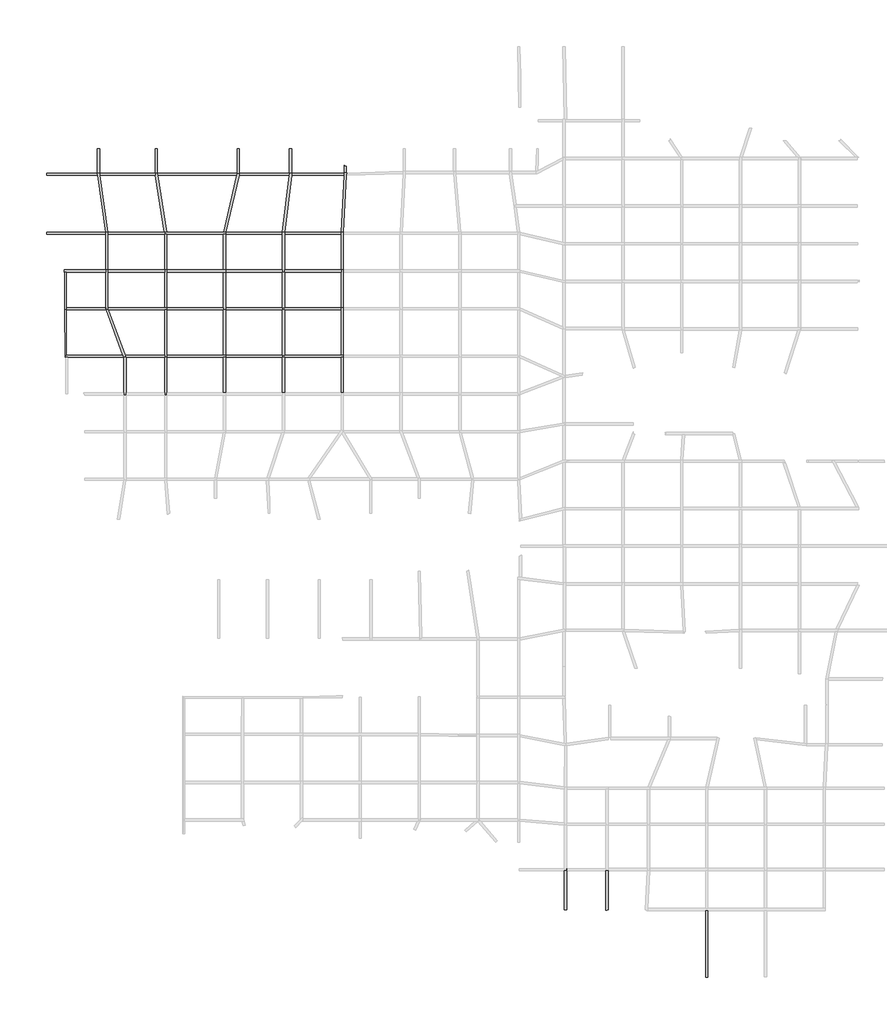
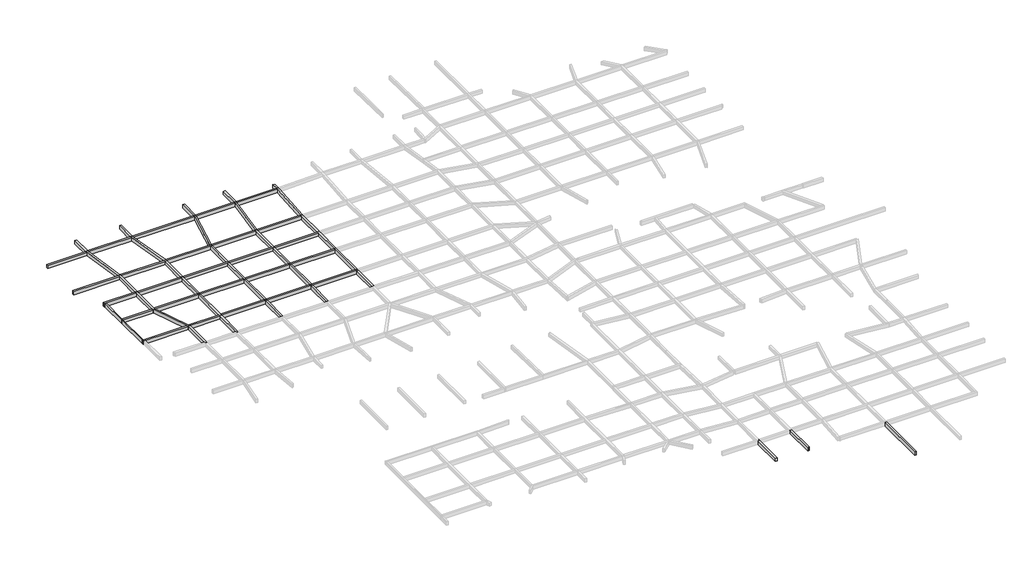
# One storey, part 2 of 15: 60 beams.
"""IFC4 building model written with IfcOpenShell, lengths in millimetres."""

from ifc_helpers import new_model, si_unit, frame, origin, place, context, project, spatial, polyline, outline, extrude, faceted_brep, element, save

model = new_model("IFC4")

# Units and contexts
model_context = context("Model", 3, world=origin())
ifc_project = project(units=[si_unit("LENGTHUNIT", "METRE", prefix="MILLI")], contexts=[model_context])

# Site, building, storey
site = spatial("IfcSite", under=ifc_project)
building = spatial("IfcBuilding", under=site)
storey = spatial("IfcBuildingStorey", under=building, Name="层高", Elevation=3300.0)

# Beams
placement = place(None, origin())
element("IfcBeam", 1, ObjectType="混凝土 - 矩形梁 : KL_beam", at=placement, inside=storey, context=model_context, shape_type="Brep", body=[
    faceted_brep([(154049.2046874, 32542.26105, 3300.0), (154049.7804968, 32392.5495084, 3300.0), (154049.7804968, 32542.26105, 3300.0), (154049.7804968, 32392.5495084, 2700.0), (154049.2046874, 32542.26105, 2700.0), (154049.7804968, 32542.26105, 2700.0)], [[[0, 1, 2]], [[3, 4, 5]], [[5, 2, 1, 3]], [[2, 5, 4, 0]], [[1, 0, 4, 3]]]),
    faceted_brep([(153749.7804968, 32242.26105, 3300.0), (153749.7804968, 32242.26105, 2700.0), (153749.7804968, 27044.9842098, 2700.0), (153749.7804968, 27044.9842098, 3300.0), (153750.3563062, 32242.26105, 3300.0), (154049.7804968, 32242.26105, 3300.0), (154049.7804968, 32242.26105, 2700.0), (153750.3563062, 32242.26105, 2700.0), (154049.7804968, 27044.9842098, 3300.0), (154049.7804968, 27044.9842098, 2700.0)], [[[0, 1, 2, 3]], [[1, 0, 4, 5, 6, 7]], [[4, 0, 3, 8, 5]], [[7, 6, 9, 2, 1]], [[6, 5, 8, 9]], [[3, 2, 9, 8]]]),
])
element("IfcBeam", 2, ObjectType="混凝土 - 矩形梁 : KL_beam", at=placement, inside=storey, context=model_context, shape_type="Brep", body=[
    faceted_brep([(159249.7804968, 32242.26105, 3300.0), (159249.7804968, 27016.5295438, 3300.0), (159372.7804968, 27016.5295438, 3300.0), (159372.7804968, 27044.9842098, 3300.0), (159492.7804968, 27044.9842098, 3300.0), (159549.7804968, 27044.9842098, 3300.0), (159549.7804968, 32242.26105, 3300.0), (159249.7804968, 27016.5295438, 2700.0), (159249.7804968, 32242.26105, 2700.0), (159549.7804968, 32242.26105, 2700.0), (159549.7804968, 27044.9842098, 2700.0), (159372.7804968, 27044.9842098, 2700.0), (159372.7804968, 27016.5295438, 2700.0)], [[[0, 1, 2, 3, 4, 5, 6]], [[7, 1, 0, 8]], [[7, 8, 9, 10, 11, 12]], [[9, 6, 5, 10]], [[0, 6, 9, 8]], [[11, 3, 2, 12]], [[3, 11, 10, 5, 4]], [[1, 7, 12, 2]]]),
])
element("IfcBeam", 3, ObjectType="混凝土 - 矩形梁 : KL_beam", at=placement, inside=storey, context=model_context, shape_type="SweptSolid", body=[
    extrude(outline(polyline([(172749.7804968, 18102.1039685), (172449.7804968, 18102.1039685), (172449.7804968, 26942.26105), (172749.7804968, 26942.26105), (172749.7804968, 18102.1039685)])), frame((0.0, 0.0, 2700.0), z_axis=(0.0, 0.0, 1.0), x_axis=(1.0, 0.0, 0.0)), (0.0, 0.0, 1.0), 600.0),
])
element("IfcBeam", 4, ObjectType="混凝土 - 矩形梁 : KL_beam", at=placement, inside=storey, context=model_context, shape_type="Brep", body=[
    faceted_brep([(92950.3009381, 106592.3894162, 3300.0), (92995.5104525, 106592.3894162, 3300.0), (93250.3009381, 106592.3894162, 3300.0), (93250.3009381, 106892.3894162, 3300.0), (93250.3009381, 111592.3894162, 3300.0), (93250.3009381, 111892.3894162, 3300.0), (92950.3009381, 111892.3894162, 3300.0), (92950.3009381, 111592.3894162, 3300.0), (92950.3009381, 106892.3894162, 3300.0), (92950.3009381, 106715.773716, 3300.0), (92950.3009381, 106592.3894162, 2700.0), (92950.3009381, 111892.3894162, 2700.0), (92950.3009381, 111592.3894162, 2700.0), (92950.3009381, 106892.3894162, 2700.0), (92950.3009381, 106715.773716, 2700.0), (93250.3009381, 106592.3894162, 2700.0), (92995.5104525, 106592.3894162, 2700.0), (93250.3009381, 111892.3894162, 2700.0), (93250.3009381, 111592.3894162, 2700.0), (93250.3009381, 106892.3894162, 2700.0)], [[[0, 1, 2, 3, 4, 5, 6, 7, 8, 9]], [[10, 0, 9, 8, 7, 6, 11, 12, 13, 14]], [[15, 16, 10, 14, 13, 12, 11, 17, 18, 19]], [[2, 15, 19, 18, 17, 5, 4, 3]], [[2, 1, 0, 10, 16, 15]], [[6, 5, 17, 11]]]),
])
element("IfcBeam", 5, ObjectType="混凝土 - 矩形梁 : KL_beam", at=placement, inside=storey, context=model_context, shape_type="Brep", body=[
    faceted_brep([(101050.3009381, 106592.3894162, 3300.0), (101050.3009381, 106892.3894162, 3300.0), (100750.3009381, 106892.3894162, 3300.0), (93250.3009381, 106892.3894162, 3300.0), (93250.3009381, 106592.3894162, 3300.0), (93315.0150877, 106592.3894162, 3300.0), (100750.3009381, 106592.3894162, 3300.0), (101050.3009381, 106592.3894162, 2700.0), (93250.3009381, 106592.3894162, 2700.0), (93315.0150877, 106592.3894162, 2700.0), (100750.3009381, 106592.3894162, 2700.0), (101050.3009381, 106892.3894162, 2700.0), (93250.3009381, 106892.3894162, 2700.0), (100750.3009381, 106892.3894162, 2700.0)], [[[0, 1, 2, 3, 4, 5, 6]], [[7, 0, 6, 5, 4, 8, 9, 10]], [[11, 7, 10, 9, 8, 12, 13]], [[1, 11, 13, 12, 3, 2]], [[4, 3, 12, 8]], [[1, 0, 7, 11]]]),
])
element("IfcBeam", 6, ObjectType="混凝土 - 矩形梁 : KL_beam", at=placement, inside=storey, context=model_context, shape_type="Brep", body=[
    faceted_brep([(101050.3009381, 111892.3894162, 3300.0), (100750.3009381, 111892.3894162, 3300.0), (100750.3009381, 111592.3894162, 3300.0), (100750.3009381, 106892.3894162, 3300.0), (101050.3009381, 106892.3894162, 3300.0), (101050.3009381, 111592.3894162, 3300.0), (101050.3009381, 111892.3894162, 2700.0), (101050.3009381, 106892.3894162, 2700.0), (101050.3009381, 111592.3894162, 2700.0), (100750.3009381, 111892.3894162, 2700.0), (100750.3009381, 106892.3894162, 2700.0), (100750.3009381, 111592.3894162, 2700.0)], [[[0, 1, 2, 3, 4, 5]], [[6, 0, 5, 4, 7, 8]], [[9, 6, 8, 7, 10, 11]], [[1, 9, 11, 10, 3, 2]], [[4, 3, 10, 7]], [[1, 0, 6, 9]]]),
])
element("IfcBeam", 7, ObjectType="混凝土 - 矩形梁 : KL_beam", at=placement, inside=storey, context=model_context, shape_type="SweptSolid", body=[
    extrude(outline(polyline([(93250.3009381, 111592.3894162), (93250.3009381, 111892.3894162), (100750.3009381, 111892.3894162), (100750.3009381, 111592.3894162), (93250.3009381, 111592.3894162)])), frame((0.0, 0.0, 2700.0), z_axis=(0.0, 0.0, 1.0), x_axis=(1.0, 0.0, 0.0)), (0.0, 0.0, 1.0), 600.0),
])
element("IfcBeam", 8, ObjectType="混凝土 - 矩形梁 : KL_beam", at=placement, inside=storey, context=model_context, shape_type="Brep", body=[
    faceted_brep([(108850.3009381, 111592.3894162, 3300.0), (108850.3009381, 111892.3894162, 3300.0), (108550.3009381, 111892.3894162, 3300.0), (101050.3009381, 111892.3894162, 3300.0), (101050.3009381, 111592.3894162, 3300.0), (108550.3009381, 111592.3894162, 3300.0), (108850.3009381, 111592.3894162, 2700.0), (101050.3009381, 111592.3894162, 2700.0), (108550.3009381, 111592.3894162, 2700.0), (108850.3009381, 111892.3894162, 2700.0), (101050.3009381, 111892.3894162, 2700.0), (108550.3009381, 111892.3894162, 2700.0)], [[[0, 1, 2, 3, 4, 5]], [[6, 0, 5, 4, 7, 8]], [[9, 6, 8, 7, 10, 11]], [[1, 9, 11, 10, 3, 2]], [[4, 3, 10, 7]], [[1, 0, 6, 9]]]),
])
element("IfcBeam", 9, ObjectType="混凝土 - 矩形梁 : KL_beam", at=placement, inside=storey, context=model_context, shape_type="Brep", body=[
    faceted_brep([(108550.3009381, 106592.3894162, 3300.0), (108850.3009381, 106592.3894162, 3300.0), (108850.3009381, 106892.3894162, 3300.0), (108850.3009381, 111592.3894162, 3300.0), (108550.3009381, 111592.3894162, 3300.0), (108550.3009381, 106892.3894162, 3300.0), (108550.3009381, 106592.3894162, 2700.0), (108550.3009381, 111592.3894162, 2700.0), (108550.3009381, 106892.3894162, 2700.0), (108850.3009381, 106592.3894162, 2700.0), (108850.3009381, 111592.3894162, 2700.0), (108850.3009381, 106892.3894162, 2700.0)], [[[0, 1, 2, 3, 4, 5]], [[6, 0, 5, 4, 7, 8]], [[9, 6, 8, 7, 10, 11]], [[1, 9, 11, 10, 3, 2]], [[4, 3, 10, 7]], [[1, 0, 6, 9]]]),
])
element("IfcBeam", 10, ObjectType="混凝土 - 矩形梁 : KL_beam", at=placement, inside=storey, context=model_context, shape_type="SweptSolid", body=[
    extrude(outline(polyline([(101050.3009381, 106592.3894162), (101050.3009381, 106892.3894162), (108550.3009381, 106892.3894162), (108550.3009381, 106592.3894162), (101050.3009381, 106592.3894162)])), frame((0.0, 0.0, 2700.0), z_axis=(0.0, 0.0, 1.0), x_axis=(1.0, 0.0, 0.0)), (0.0, 0.0, 1.0), 600.0),
])
element("IfcBeam", 11, ObjectType="混凝土 - 矩形梁 : KL_beam", at=placement, inside=storey, context=model_context, shape_type="Brep", body=[
    faceted_brep([(100750.3009381, 100292.3894162, 3300.0), (101050.3009381, 100292.3894162, 3300.0), (101050.3009381, 100592.3894162, 3300.0), (101050.3009381, 106592.3894162, 3300.0), (100750.3009381, 106592.3894162, 3300.0), (100750.3009381, 100592.3894162, 3300.0), (101050.3009381, 100292.3894162, 2700.0), (101050.3009381, 100592.3894162, 2700.0), (101050.3009381, 106592.3894162, 2700.0), (100750.3009381, 100292.3894162, 2700.0), (100750.3009381, 100592.3894162, 2700.0), (100750.3009381, 106592.3894162, 2700.0)], [[[0, 1, 2, 3, 4, 5]], [[1, 6, 7, 8, 3, 2]], [[6, 9, 10, 11, 8, 7]], [[9, 0, 5, 4, 11, 10]], [[4, 3, 8, 11]], [[1, 0, 9, 6]]]),
])
element("IfcBeam", 12, ObjectType="混凝土 - 矩形梁 : KL_beam", at=placement, inside=storey, context=model_context, shape_type="Brep", body=[
    faceted_brep([(92950.3009381, 106715.773716, 3300.0), (92950.3009381, 106892.3894162, 3300.0), (92885.5867885, 106892.3894162, 3300.0), (92950.3009381, 106892.3894162, 2700.0), (92950.3009381, 106715.773716, 2700.0), (92885.5867885, 106892.3894162, 2700.0)], [[[0, 1, 2]], [[3, 4, 5]], [[2, 5, 4, 0]], [[5, 2, 1, 3]], [[1, 0, 4, 3]]]),
    faceted_brep([(95623.4120324, 100292.3894162, 3300.0), (95623.4120324, 100292.3894162, 2700.0), (95513.4883684, 100592.3894162, 2700.0), (93315.0150877, 106592.3894162, 2700.0), (93315.0150877, 106592.3894162, 3300.0), (95513.4883684, 100592.3894162, 3300.0), (93250.3009381, 106592.3894162, 2700.0), (92995.5104525, 106592.3894162, 2700.0), (92995.5104525, 106592.3894162, 3300.0), (93250.3009381, 106592.3894162, 3300.0), (95350.3009362, 100292.3894162, 3300.0), (95303.9073972, 100292.3894162, 3300.0), (95303.9073972, 100292.3894162, 2700.0), (95350.3009362, 100292.3894162, 2700.0), (95193.9837332, 100592.3894162, 3300.0), (95193.9837332, 100592.3894162, 2700.0)], [[[0, 1, 2, 3, 4, 5]], [[4, 3, 6, 7, 8, 9]], [[0, 10, 11, 12, 13, 1]], [[4, 9, 8, 14, 11, 10, 0, 5]], [[7, 6, 3, 2, 1, 13, 12, 15]], [[8, 7, 15, 12, 11, 14]]]),
])
element("IfcBeam", 13, ObjectType="混凝土 - 矩形梁 : KL_beam", at=placement, inside=storey, context=model_context, shape_type="Brep", body=[
    faceted_brep([(100750.3009381, 100292.3894162, 3300.0), (100750.3009381, 100592.3894162, 3300.0), (95513.4883684, 100592.3894162, 3300.0), (95623.4120324, 100292.3894162, 3300.0), (95650.3009362, 100292.3894162, 3300.0), (100750.3009381, 100292.3894162, 2700.0), (95623.4120324, 100292.3894162, 2700.0), (95650.3009362, 100292.3894162, 2700.0), (100750.3009381, 100592.3894162, 2700.0), (95513.4883684, 100592.3894162, 2700.0)], [[[0, 1, 2, 3, 4]], [[5, 0, 4, 3, 6, 7]], [[8, 5, 7, 6, 9]], [[1, 8, 9, 2]], [[1, 0, 5, 8]], [[3, 2, 9, 6]]]),
])
element("IfcBeam", 14, ObjectType="混凝土 - 矩形梁 : KL_beam", at=placement, inside=storey, context=model_context, shape_type="Brep", body=[
    faceted_brep([(108850.3009381, 100292.3894162, 3300.0), (108850.3009381, 100592.3894162, 3300.0), (108550.3009381, 100592.3894162, 3300.0), (101050.3009381, 100592.3894162, 3300.0), (101050.3009381, 100292.3894162, 3300.0), (108550.3009381, 100292.3894162, 3300.0), (108850.3009381, 100592.3894162, 2700.0), (108550.3009381, 100592.3894162, 2700.0), (101050.3009381, 100592.3894162, 2700.0), (108850.3009381, 100292.3894162, 2700.0), (108550.3009381, 100292.3894162, 2700.0), (101050.3009381, 100292.3894162, 2700.0)], [[[0, 1, 2, 3, 4, 5]], [[1, 6, 7, 8, 3, 2]], [[6, 9, 10, 11, 8, 7]], [[9, 0, 5, 4, 11, 10]], [[4, 3, 8, 11]], [[1, 0, 9, 6]]]),
])
element("IfcBeam", 15, ObjectType="混凝土 - 矩形梁 : KL_beam", at=placement, inside=storey, context=model_context, shape_type="SweptSolid", body=[
    extrude(outline(polyline([(108550.3009381, 106592.3894162), (108850.3009381, 106592.3894162), (108850.3009381, 100592.3894162), (108550.3009381, 100592.3894162), (108550.3009381, 106592.3894162)])), frame((0.0, 0.0, 2700.0), z_axis=(0.0, 0.0, 1.0), x_axis=(1.0, 0.0, 0.0)), (0.0, 0.0, 1.0), 600.0),
])
element("IfcBeam", 16, ObjectType="混凝土 - 矩形梁 : KL_beam", at=placement, inside=storey, context=model_context, shape_type="Brep", body=[
    faceted_brep([(100750.3009381, 95292.1233035, 3300.0), (101050.3009381, 95292.1233035, 3300.0), (101050.3009381, 95592.1233035, 3300.0), (101050.3009381, 100292.3894162, 3300.0), (100750.3009381, 100292.3894162, 3300.0), (100750.3009381, 95592.1233035, 3300.0), (101050.3009381, 95292.1233035, 2700.0), (101050.3009381, 95592.1233035, 2700.0), (101050.3009381, 100292.3894162, 2700.0), (100750.3009381, 95292.1233035, 2700.0), (100750.3009381, 95592.1233035, 2700.0), (100750.3009381, 100292.3894162, 2700.0)], [[[0, 1, 2, 3, 4, 5]], [[1, 6, 7, 8, 3, 2]], [[6, 9, 10, 11, 8, 7]], [[9, 0, 5, 4, 11, 10]], [[4, 3, 8, 11]], [[1, 0, 9, 6]]]),
])
element("IfcBeam", 17, ObjectType="混凝土 - 矩形梁 : KL_beam", at=placement, inside=storey, context=model_context, shape_type="Brep", body=[
    faceted_brep([(95350.3009362, 95292.1233035, 3300.0), (95650.3009362, 95292.1233035, 3300.0), (95650.3009362, 95592.1233035, 3300.0), (95650.3009362, 100292.3894162, 3300.0), (95623.4120324, 100292.3894162, 3300.0), (95350.3009362, 100292.3894162, 3300.0), (95350.3009362, 95567.3846604, 3300.0), (95650.3009362, 95292.1233035, 2700.0), (95650.3009362, 95592.1233035, 2700.0), (95650.3009362, 100292.3894162, 2700.0), (95350.3009362, 95292.1233035, 2700.0), (95350.3009362, 95567.3846604, 2700.0), (95350.3009362, 100292.3894162, 2700.0), (95623.4120324, 100292.3894162, 2700.0)], [[[0, 1, 2, 3, 4, 5, 6]], [[1, 7, 8, 9, 3, 2]], [[7, 10, 11, 12, 13, 9, 8]], [[10, 0, 6, 5, 12, 11]], [[5, 4, 3, 9, 13, 12]], [[1, 0, 10, 7]]]),
])
element("IfcBeam", 18, ObjectType="混凝土 - 矩形梁 : KL_beam", at=placement, inside=storey, context=model_context, shape_type="SweptSolid", body=[
    extrude(outline(polyline([(108550.3009381, 100292.3894162), (108850.3009381, 100292.3894162), (108850.3009381, 95592.1233035), (108550.3009381, 95592.1233035), (108550.3009381, 100292.3894162)])), frame((0.0, 0.0, 2700.0), z_axis=(0.0, 0.0, 1.0), x_axis=(1.0, 0.0, 0.0)), (0.0, 0.0, 1.0), 600.0),
])
element("IfcBeam", 19, ObjectType="混凝土 - 矩形梁 : KL_beam", at=placement, inside=storey, context=model_context, shape_type="Brep", body=[
    faceted_brep([(87611.9695307, 100592.3894162, 3300.0), (87614.7715216, 100292.3894162, 3300.0), (87650.3009381, 100292.3894162, 3300.0), (87950.3009381, 100292.3894162, 3300.0), (95303.9073972, 100292.3894162, 3300.0), (95193.9837332, 100592.3894162, 3300.0), (87750.3009381, 100592.3894162, 3300.0), (87611.9695307, 100592.3894162, 2700.0), (95193.9837332, 100592.3894162, 2700.0), (87750.3009381, 100592.3894162, 2700.0), (87614.7715216, 100292.3894162, 2700.0), (95303.9073972, 100292.3894162, 2700.0), (87950.3009381, 100292.3894162, 2700.0), (87650.3009381, 100292.3894162, 2700.0)], [[[0, 1, 2, 3, 4, 5, 6]], [[7, 0, 6, 5, 8, 9]], [[10, 7, 9, 8, 11, 12, 13]], [[1, 10, 13, 12, 11, 4, 3, 2]], [[1, 0, 7, 10]], [[5, 4, 11, 8]]]),
])
element("IfcBeam", 20, ObjectType="混凝土 - 矩形梁 : KL_beam", at=placement, inside=storey, context=model_context, shape_type="Brep", body=[
    faceted_brep([(124450.3009381, 100292.3894162, 3300.0), (124450.3009381, 100592.3894162, 3300.0), (124150.3009381, 100592.3894162, 3300.0), (116650.3009381, 100592.3894162, 3300.0), (116350.3009381, 100592.3894162, 3300.0), (116350.3009381, 100292.3894162, 3300.0), (116650.3009381, 100292.3894162, 3300.0), (124150.3009381, 100292.3894162, 3300.0), (124450.3009381, 100292.3894162, 2700.0), (116350.3009381, 100292.3894162, 2700.0), (116650.3009381, 100292.3894162, 2700.0), (124150.3009381, 100292.3894162, 2700.0), (124450.3009381, 100592.3894162, 2700.0), (116350.3009381, 100592.3894162, 2700.0), (116650.3009381, 100592.3894162, 2700.0), (124150.3009381, 100592.3894162, 2700.0)], [[[0, 1, 2, 3, 4, 5, 6, 7]], [[8, 0, 7, 6, 5, 9, 10, 11]], [[12, 8, 11, 10, 9, 13, 14, 15]], [[1, 12, 15, 14, 13, 4, 3, 2]], [[1, 0, 8, 12]], [[5, 4, 13, 9]]]),
])
element("IfcBeam", 21, ObjectType="混凝土 - 矩形梁 : KL_beam", at=placement, inside=storey, context=model_context, shape_type="Brep", body=[
    faceted_brep([(124450.3009381, 106892.3894162, 3300.0), (124150.3009381, 106892.3894162, 3300.0), (124150.3009381, 106592.3894162, 3300.0), (124150.3009381, 100592.3894162, 3300.0), (124450.3009381, 100592.3894162, 3300.0), (124450.3009381, 106592.3894162, 3300.0), (124450.3009381, 106892.3894162, 2700.0), (124450.3009381, 100592.3894162, 2700.0), (124450.3009381, 106592.3894162, 2700.0), (124150.3009381, 106892.3894162, 2700.0), (124150.3009381, 100592.3894162, 2700.0), (124150.3009381, 106592.3894162, 2700.0)], [[[0, 1, 2, 3, 4, 5]], [[6, 0, 5, 4, 7, 8]], [[9, 6, 8, 7, 10, 11]], [[1, 9, 11, 10, 3, 2]], [[4, 3, 10, 7]], [[1, 0, 6, 9]]]),
])
element("IfcBeam", 22, ObjectType="混凝土 - 矩形梁 : KL_beam", at=placement, inside=storey, context=model_context, shape_type="Brep", body=[
    faceted_brep([(116350.3009381, 106892.3894162, 3300.0), (116350.3009381, 106592.3894162, 3300.0), (116650.3009381, 106592.3894162, 3300.0), (124150.3009381, 106592.3894162, 3300.0), (124150.3009381, 106892.3894162, 3300.0), (116650.3009381, 106892.3894162, 3300.0), (116350.3009381, 106892.3894162, 2700.0), (124150.3009381, 106892.3894162, 2700.0), (116650.3009381, 106892.3894162, 2700.0), (116350.3009381, 106592.3894162, 2700.0), (124150.3009381, 106592.3894162, 2700.0), (116650.3009381, 106592.3894162, 2700.0)], [[[0, 1, 2, 3, 4, 5]], [[6, 0, 5, 4, 7, 8]], [[9, 6, 8, 7, 10, 11]], [[1, 9, 11, 10, 3, 2]], [[4, 3, 10, 7]], [[1, 0, 6, 9]]]),
])
element("IfcBeam", 23, ObjectType="混凝土 - 矩形梁 : KL_beam", at=placement, inside=storey, context=model_context, shape_type="SweptSolid", body=[
    extrude(outline(polyline([(116650.3009381, 100592.3894162), (116350.3009381, 100592.3894162), (116350.3009381, 106592.3894162), (116650.3009381, 106592.3894162), (116650.3009381, 100592.3894162)])), frame((0.0, 0.0, 2700.0), z_axis=(0.0, 0.0, 1.0), x_axis=(1.0, 0.0, 0.0)), (0.0, 0.0, 1.0), 600.0),
])
element("IfcBeam", 24, ObjectType="混凝土 - 矩形梁 : KL_beam", at=placement, inside=storey, context=model_context, shape_type="SweptSolid", body=[
    extrude(outline(polyline([(116350.3009381, 100292.3894162), (116650.3009381, 100292.3894162), (116650.3009381, 95592.1233035), (116350.3009381, 95592.1233035), (116350.3009381, 100292.3894162)])), frame((0.0, 0.0, 2700.0), z_axis=(0.0, 0.0, 1.0), x_axis=(1.0, 0.0, 0.0)), (0.0, 0.0, 1.0), 600.0),
])
element("IfcBeam", 25, ObjectType="混凝土 - 矩形梁 : KL_beam", at=placement, inside=storey, context=model_context, shape_type="SweptSolid", body=[
    extrude(outline(polyline([(124150.3009381, 100292.3894162), (124450.3009381, 100292.3894162), (124450.3009381, 95592.1233035), (124150.3009381, 95592.1233035), (124150.3009381, 100292.3894162)])), frame((0.0, 0.0, 2700.0), z_axis=(0.0, 0.0, 1.0), x_axis=(1.0, 0.0, 0.0)), (0.0, 0.0, 1.0), 600.0),
])
element("IfcBeam", 26, ObjectType="混凝土 - 矩形梁 : KL_beam", at=placement, inside=storey, context=model_context, shape_type="Brep", body=[
    faceted_brep([(116350.3009381, 111592.3894162, 3300.0), (116650.3009381, 111592.3894162, 3300.0), (116650.3009381, 111892.3894162, 3300.0), (116650.3009381, 116592.3894162, 3300.0), (116650.3009381, 116892.3894162, 3300.0), (116367.5921484, 116892.3894162, 3300.0), (116350.3009381, 116892.3894162, 3300.0), (116350.3009381, 116592.3894162, 3300.0), (116350.3009381, 111892.3894162, 3300.0), (116350.3009381, 111592.3894162, 2700.0), (116350.3009381, 116892.3894162, 2700.0), (116350.3009381, 116592.3894162, 2700.0), (116350.3009381, 111892.3894162, 2700.0), (116650.3009381, 111592.3894162, 2700.0), (116367.5921484, 116892.3894162, 2700.0), (116650.3009381, 116892.3894162, 2700.0), (116650.3009381, 116592.3894162, 2700.0), (116650.3009381, 111892.3894162, 2700.0)], [[[0, 1, 2, 3, 4, 5, 6, 7, 8]], [[9, 0, 8, 7, 6, 10, 11, 12]], [[13, 9, 12, 11, 10, 14, 15, 16, 17]], [[1, 13, 17, 16, 15, 4, 3, 2]], [[1, 0, 9, 13]], [[6, 5, 4, 15, 14, 10]]]),
])
element("IfcBeam", 27, ObjectType="混凝土 - 矩形梁 : KL_beam", at=placement, inside=storey, context=model_context, shape_type="SweptSolid", body=[
    extrude(outline(polyline([(116650.3009381, 106892.3894162), (116350.3009381, 106892.3894162), (116350.3009381, 111592.3894162), (116650.3009381, 111592.3894162), (116650.3009381, 106892.3894162)])), frame((0.0, 0.0, 2700.0), z_axis=(0.0, 0.0, 1.0), x_axis=(1.0, 0.0, 0.0)), (0.0, 0.0, 1.0), 600.0),
])
element("IfcBeam", 28, ObjectType="混凝土 - 矩形梁 : KL_beam", at=placement, inside=storey, context=model_context, shape_type="Brep", body=[
    faceted_brep([(124450.3009381, 111892.3894162, 3300.0), (124150.3009381, 111892.3894162, 3300.0), (124150.3009381, 111592.3894162, 3300.0), (124150.3009381, 106892.3894162, 3300.0), (124450.3009381, 106892.3894162, 3300.0), (124450.3009381, 111592.3894162, 3300.0), (124150.3009381, 111892.3894162, 2700.0), (124150.3009381, 111592.3894162, 2700.0), (124150.3009381, 106892.3894162, 2700.0), (124450.3009381, 111892.3894162, 2700.0), (124450.3009381, 111592.3894162, 2700.0), (124450.3009381, 106892.3894162, 2700.0)], [[[0, 1, 2, 3, 4, 5]], [[1, 6, 7, 8, 3, 2]], [[6, 9, 10, 11, 8, 7]], [[9, 0, 5, 4, 11, 10]], [[4, 3, 8, 11]], [[1, 0, 9, 6]]]),
])
element("IfcBeam", 29, ObjectType="混凝土 - 矩形梁 : KL_beam", at=placement, inside=storey, context=model_context, shape_type="SweptSolid", body=[
    extrude(outline(polyline([(116650.3009381, 111592.3894162), (116650.3009381, 111892.3894162), (124150.3009381, 111892.3894162), (124150.3009381, 111592.3894162), (116650.3009381, 111592.3894162)])), frame((0.0, 0.0, 2700.0), z_axis=(0.0, 0.0, 1.0), x_axis=(1.0, 0.0, 0.0)), (0.0, 0.0, 1.0), 600.0),
])
element("IfcBeam", 30, ObjectType="混凝土 - 矩形梁 : KL_beam", at=placement, inside=storey, context=model_context, shape_type="Brep", body=[
    faceted_brep([(124450.3009381, 116892.3894162, 3300.0), (124157.9562531, 116892.3894162, 3300.0), (124150.3009381, 116892.3894162, 3300.0), (124150.3009381, 116592.3894162, 3300.0), (124150.3009381, 111892.3894162, 3300.0), (124450.3009381, 111892.3894162, 3300.0), (124450.3009381, 116592.3894162, 3300.0), (124450.3009381, 116738.461528, 3300.0), (124450.3009381, 116892.3894162, 2700.0), (124450.3009381, 111892.3894162, 2700.0), (124450.3009381, 116592.3894162, 2700.0), (124450.3009381, 116738.461528, 2700.0), (124150.3009381, 116892.3894162, 2700.0), (124157.9562531, 116892.3894162, 2700.0), (124150.3009381, 111892.3894162, 2700.0), (124150.3009381, 116592.3894162, 2700.0)], [[[0, 1, 2, 3, 4, 5, 6, 7]], [[8, 0, 7, 6, 5, 9, 10, 11]], [[12, 13, 8, 11, 10, 9, 14, 15]], [[2, 12, 15, 14, 4, 3]], [[5, 4, 14, 9]], [[2, 1, 0, 8, 13, 12]]]),
])
element("IfcBeam", 31, ObjectType="混凝土 - 矩形梁 : KL_beam", at=placement, inside=storey, context=model_context, shape_type="Brep", body=[
    faceted_brep([(116650.3009381, 116892.3894162, 3300.0), (116650.3009381, 116592.3894162, 3300.0), (124150.3009381, 116592.3894162, 3300.0), (124150.3009381, 116892.3894162, 3300.0), (116669.8450961, 116892.3894162, 3300.0), (116650.3009381, 116892.3894162, 2700.0), (124150.3009381, 116892.3894162, 2700.0), (116669.8450961, 116892.3894162, 2700.0), (116650.3009381, 116592.3894162, 2700.0), (124150.3009381, 116592.3894162, 2700.0)], [[[0, 1, 2, 3, 4]], [[5, 0, 4, 3, 6, 7]], [[8, 5, 7, 6, 9]], [[1, 8, 9, 2]], [[1, 0, 5, 8]], [[3, 2, 9, 6]]]),
])
element("IfcBeam", 32, ObjectType="混凝土 - 矩形梁 : KL_beam", at=placement, inside=storey, context=model_context, shape_type="Brep", body=[
    faceted_brep([(100750.3009381, 116892.3894162, 3300.0), (100750.3009381, 116592.3894162, 3300.0), (101050.3009381, 116592.3894162, 3300.0), (108550.3009381, 116592.3894162, 3300.0), (108850.3009381, 116592.3894162, 3300.0), (108850.3009381, 116892.3894162, 3300.0), (108580.9855506, 116892.3894162, 3300.0), (101028.4130409, 116892.3894162, 3300.0), (100750.3009381, 116592.3894162, 2700.0), (101050.3009381, 116592.3894162, 2700.0), (108550.3009381, 116592.3894162, 2700.0), (108850.3009381, 116592.3894162, 2700.0), (100750.3009381, 116892.3894162, 2700.0), (101028.4130409, 116892.3894162, 2700.0), (108580.9855506, 116892.3894162, 2700.0), (108850.3009381, 116892.3894162, 2700.0)], [[[0, 1, 2, 3, 4, 5, 6, 7]], [[1, 8, 9, 10, 11, 4, 3, 2]], [[8, 12, 13, 14, 15, 11, 10, 9]], [[12, 0, 7, 6, 5, 15, 14, 13]], [[1, 0, 12, 8]], [[5, 4, 11, 15]]]),
])
element("IfcBeam", 33, ObjectType="混凝土 - 矩形梁 : KL_beam", at=placement, inside=storey, context=model_context, shape_type="SweptSolid", body=[
    extrude(outline(polyline([(101050.3009381, 111892.3894162), (100750.3009381, 111892.3894162), (100750.3009381, 116592.3894162), (101050.3009381, 116592.3894162), (101050.3009381, 111892.3894162)])), frame((0.0, 0.0, 2700.0), z_axis=(0.0, 0.0, 1.0), x_axis=(1.0, 0.0, 0.0)), (0.0, 0.0, 1.0), 600.0),
])
element("IfcBeam", 34, ObjectType="混凝土 - 矩形梁 : KL_beam", at=placement, inside=storey, context=model_context, shape_type="SweptSolid", body=[
    extrude(outline(polyline([(108850.3009381, 111892.3894162), (108550.3009381, 111892.3894162), (108550.3009381, 116592.3894162), (108850.3009381, 116592.3894162), (108850.3009381, 111892.3894162)])), frame((0.0, 0.0, 2700.0), z_axis=(0.0, 0.0, 1.0), x_axis=(1.0, 0.0, 0.0)), (0.0, 0.0, 1.0), 600.0),
])
element("IfcBeam", 35, ObjectType="混凝土 - 矩形梁 : KL_beam", at=placement, inside=storey, context=model_context, shape_type="Brep", body=[
    faceted_brep([(93250.3009381, 116892.3894162, 3300.0), (93230.6939488, 116892.3894162, 3300.0), (92950.3009381, 116892.3894162, 3300.0), (92950.3009381, 116592.3894162, 3300.0), (92950.3009381, 111892.3894162, 3300.0), (93250.3009381, 111892.3894162, 3300.0), (93250.3009381, 116592.3894162, 3300.0), (92950.3009381, 116892.3894162, 2700.0), (92950.3009381, 116592.3894162, 2700.0), (92950.3009381, 111892.3894162, 2700.0), (93230.6939488, 116892.3894162, 2700.0), (93250.3009381, 116892.3894162, 2700.0), (93250.3009381, 116592.3894162, 2700.0), (93250.3009381, 111892.3894162, 2700.0)], [[[0, 1, 2, 3, 4, 5, 6]], [[2, 7, 8, 9, 4, 3]], [[7, 10, 11, 12, 13, 9, 8]], [[11, 0, 6, 5, 13, 12]], [[5, 4, 9, 13]], [[2, 1, 0, 11, 10, 7]]]),
])
element("IfcBeam", 36, ObjectType="混凝土 - 矩形梁 : KL_beam", at=placement, inside=storey, context=model_context, shape_type="Brep", body=[
    faceted_brep([(100750.3009381, 116592.3894162, 3300.0), (100750.3009381, 116892.3894162, 3300.0), (100724.6735032, 116892.3894162, 3300.0), (93250.3009381, 116892.3894162, 3300.0), (93250.3009381, 116592.3894162, 3300.0), (100750.3009381, 116592.3894162, 2700.0), (93250.3009381, 116592.3894162, 2700.0), (100750.3009381, 116892.3894162, 2700.0), (93250.3009381, 116892.3894162, 2700.0), (100724.6735032, 116892.3894162, 2700.0)], [[[0, 1, 2, 3, 4]], [[5, 0, 4, 6]], [[7, 5, 6, 8, 9]], [[1, 7, 9, 8, 3, 2]], [[1, 0, 5, 7]], [[4, 3, 8, 6]]]),
])
element("IfcBeam", 37, ObjectType="混凝土 - 矩形梁 : KL_beam", at=placement, inside=storey, context=model_context, shape_type="Brep", body=[
    faceted_brep([(87450.3009381, 111892.3894162, 3300.0), (87450.3009381, 111592.3894162, 3300.0), (87750.3009381, 111592.3894162, 3300.0), (92950.3009381, 111592.3894162, 3300.0), (92950.3009381, 111892.3894162, 3300.0), (87450.3009381, 111892.3894162, 2700.0), (92950.3009381, 111892.3894162, 2700.0), (87450.3009381, 111592.3894162, 2700.0), (92950.3009381, 111592.3894162, 2700.0), (87750.3009381, 111592.3894162, 2700.0)], [[[0, 1, 2, 3, 4]], [[5, 0, 4, 6]], [[7, 5, 6, 8, 9]], [[1, 7, 9, 8, 3, 2]], [[4, 3, 8, 6]], [[1, 0, 5, 7]]]),
])
element("IfcBeam", 38, ObjectType="混凝土 - 矩形梁 : KL_beam", at=placement, inside=storey, context=model_context, shape_type="Brep", body=[
    faceted_brep([(87750.3009381, 111592.3894162, 3300.0), (87450.3009381, 111592.3894162, 3300.0), (87450.3009381, 111537.3894148, 3300.0), (87509.7435642, 111537.3894148, 3300.0), (87555.9297135, 106592.3894162, 3300.0), (87750.3009381, 106592.3894162, 3300.0), (87750.3009381, 106892.3894162, 3300.0), (87450.3009381, 111592.3894162, 2700.0), (87450.3009381, 111537.3894148, 2700.0), (87750.3009381, 111592.3894162, 2700.0), (87750.3009381, 106892.3894162, 2700.0), (87750.3009381, 106592.3894162, 2700.0), (87555.9297135, 106592.3894162, 2700.0), (87509.7435642, 111537.3894148, 2700.0)], [[[0, 1, 2, 3, 4, 5, 6]], [[1, 7, 8, 2]], [[7, 9, 10, 11, 12, 13, 8]], [[9, 0, 6, 5, 11, 10]], [[1, 0, 9, 7]], [[3, 13, 12, 4]], [[13, 3, 2, 8]], [[11, 5, 4, 12]]]),
])
element("IfcBeam", 39, ObjectType="混凝土 - 矩形梁 : KL_beam", at=placement, inside=storey, context=model_context, shape_type="SweptSolid", body=[
    extrude(outline(polyline([(92950.3009381, 106715.773716), (92950.3009381, 106592.3894162), (87750.3009381, 106592.3894162), (87750.3009381, 106892.3894162), (92885.5867885, 106892.3894162), (92950.3009381, 106715.773716)])), frame((0.0, 0.0, 2700.0), z_axis=(0.0, 0.0, 1.0), x_axis=(1.0, 0.0, 0.0)), (0.0, 0.0, 1.0), 600.0),
])
element("IfcBeam", 40, ObjectType="混凝土 - 矩形梁 : KL_beam", at=placement, inside=storey, context=model_context, shape_type="SweptSolid", body=[
    extrude(outline(polyline([(87750.3009381, 106592.3894162), (87750.3009381, 100592.3894162), (87611.9695307, 100592.3894162), (87555.9297135, 106592.3894162), (87750.3009381, 106592.3894162)])), frame((0.0, 0.0, 2700.0), z_axis=(0.0, 0.0, 1.0), x_axis=(1.0, 0.0, 0.0)), (0.0, 0.0, 1.0), 600.0),
])
element("IfcBeam", 41, ObjectType="混凝土 - 矩形梁 : KL_beam", at=placement, inside=storey, context=model_context, shape_type="SweptSolid", body=[
    extrude(outline(polyline([(108850.3009381, 100292.3894162), (108850.3009381, 100592.3894162), (116350.3009381, 100592.3894162), (116350.3009381, 100292.3894162), (108850.3009381, 100292.3894162)])), frame((0.0, 0.0, 2700.0), z_axis=(0.0, 0.0, 1.0), x_axis=(1.0, 0.0, 0.0)), (0.0, 0.0, 1.0), 600.0),
])
element("IfcBeam", 42, ObjectType="混凝土 - 矩形梁 : KL_beam", at=placement, inside=storey, context=model_context, shape_type="SweptSolid", body=[
    extrude(outline(polyline([(108850.3009381, 106592.3894162), (108850.3009381, 106892.3894162), (116350.3009381, 106892.3894162), (116350.3009381, 106592.3894162), (108850.3009381, 106592.3894162)])), frame((0.0, 0.0, 2700.0), z_axis=(0.0, 0.0, 1.0), x_axis=(1.0, 0.0, 0.0)), (0.0, 0.0, 1.0), 600.0),
])
element("IfcBeam", 43, ObjectType="混凝土 - 矩形梁 : KL_beam", at=placement, inside=storey, context=model_context, shape_type="SweptSolid", body=[
    extrude(outline(polyline([(108850.3009381, 111592.3894162), (108850.3009381, 111892.3894162), (116350.3009381, 111892.3894162), (116350.3009381, 111592.3894162), (108850.3009381, 111592.3894162)])), frame((0.0, 0.0, 2700.0), z_axis=(0.0, 0.0, 1.0), x_axis=(1.0, 0.0, 0.0)), (0.0, 0.0, 1.0), 600.0),
])
element("IfcBeam", 44, ObjectType="混凝土 - 矩形梁 : KL_beam", at=placement, inside=storey, context=model_context, shape_type="Brep", body=[
    faceted_brep([(116350.3009381, 116592.3894162, 3300.0), (116350.3009381, 116892.3894162, 3300.0), (108888.876783, 116892.3894162, 3300.0), (108850.3009381, 116892.3894162, 3300.0), (108850.3009381, 116592.3894162, 3300.0), (116350.3009381, 116892.3894162, 2700.0), (108888.876783, 116892.3894162, 2700.0), (108850.3009381, 116892.3894162, 2700.0), (116350.3009381, 116592.3894162, 2700.0), (108850.3009381, 116592.3894162, 2700.0)], [[[0, 1, 2, 3, 4]], [[1, 5, 6, 7, 3, 2]], [[5, 8, 9, 7, 6]], [[8, 0, 4, 9]], [[1, 0, 8, 5]], [[4, 3, 7, 9]]]),
])
element("IfcBeam", 45, ObjectType="混凝土 - 矩形梁 : KL_beam", at=placement, inside=storey, context=model_context, shape_type="Brep", body=[
    faceted_brep([(85110.3013454, 116892.3894162, 3300.0), (85110.3013454, 116592.3894162, 3300.0), (92950.3009381, 116592.3894162, 3300.0), (92950.3009381, 116892.3894162, 3300.0), (92927.745677, 116892.3894162, 3300.0), (85110.3013454, 116892.3894162, 2700.0), (92950.3009381, 116892.3894162, 2700.0), (92927.745677, 116892.3894162, 2700.0), (85110.3013454, 116592.3894162, 2700.0), (92950.3009381, 116592.3894162, 2700.0)], [[[0, 1, 2, 3, 4]], [[5, 0, 4, 3, 6, 7]], [[8, 5, 7, 6, 9]], [[1, 8, 9, 2]], [[1, 0, 5, 8]], [[3, 2, 9, 6]]]),
])
element("IfcBeam", 46, ObjectType="混凝土 - 矩形梁 : KL_beam", at=placement, inside=storey, context=model_context, shape_type="Brep", body=[
    faceted_brep([(92927.745677, 116892.3894162, 3300.0), (92950.3009381, 116892.3894162, 3300.0), (93230.6939488, 116892.3894162, 3300.0), (92173.3887016, 124415.5071593, 3300.0), (92131.2264512, 124715.5071593, 3300.0), (91850.8334405, 124676.1004915, 3300.0), (91834.1460306, 124673.755229, 3300.0), (91850.8334405, 124555.0181375, 3300.0), (91870.4404299, 124415.5071593, 3300.0), (93230.6939488, 116892.3894162, 2700.0), (92173.3887016, 124415.5071593, 2700.0), (92131.2264512, 124715.5071593, 2700.0), (92950.3009381, 116892.3894162, 2700.0), (92927.745677, 116892.3894162, 2700.0), (91870.4404299, 124415.5071593, 2700.0), (91850.8334405, 124555.0181375, 2700.0), (91834.1460306, 124673.755229, 2700.0), (91850.8334405, 124676.1004915, 2700.0)], [[[0, 1, 2, 3, 4, 5, 6, 7, 8]], [[4, 3, 2, 9, 10, 11]], [[11, 10, 9, 12, 13, 14, 15, 16, 17]], [[6, 16, 15, 14, 13, 0, 8, 7]], [[0, 13, 12, 9, 2, 1]], [[6, 5, 4, 11, 17, 16]]]),
])
element("IfcBeam", 47, ObjectType="混凝土 - 矩形梁 : KL_beam", at=placement, inside=storey, context=model_context, shape_type="Brep", body=[
    faceted_brep([(100724.6735032, 116892.3894162, 3300.0), (100750.3009381, 116892.3894162, 3300.0), (101028.4130409, 116892.3894162, 3300.0), (99836.8682477, 124415.5071593, 3300.0), (99789.3529156, 124715.5071593, 3300.0), (99511.2408128, 124715.5071593, 3300.0), (99485.6133779, 124715.5071593, 3300.0), (99533.12871, 124415.5071593, 3300.0), (101028.4130409, 116892.3894162, 2700.0), (99836.8682477, 124415.5071593, 2700.0), (99789.3529156, 124715.5071593, 2700.0), (100750.3009381, 116892.3894162, 2700.0), (100724.6735032, 116892.3894162, 2700.0), (99533.12871, 124415.5071593, 2700.0), (99485.6133779, 124715.5071593, 2700.0), (99511.2408128, 124715.5071593, 2700.0)], [[[0, 1, 2, 3, 4, 5, 6, 7]], [[2, 8, 9, 10, 4, 3]], [[8, 11, 12, 13, 14, 15, 10, 9]], [[6, 14, 13, 12, 0, 7]], [[0, 12, 11, 8, 2, 1]], [[6, 5, 4, 10, 15, 14]]]),
])
element("IfcBeam", 48, ObjectType="混凝土 - 矩形梁 : KL_beam", at=placement, inside=storey, context=model_context, shape_type="Brep", body=[
    faceted_brep([(110387.0945929, 124715.5071593, 3300.0), (110317.8341356, 124415.5071593, 3300.0), (108580.9855506, 116892.3894162, 3300.0), (108850.3009381, 116892.3894162, 3300.0), (108888.876783, 116892.3894162, 3300.0), (110625.7253679, 124415.5071593, 3300.0), (110679.4056124, 124648.021843, 3300.0), (110679.4056124, 124648.021843, 2700.0), (108888.876783, 116892.3894162, 2700.0), (110625.7253679, 124415.5071593, 2700.0), (108850.3009381, 116892.3894162, 2700.0), (108580.9855506, 116892.3894162, 2700.0), (110317.8341356, 124415.5071593, 2700.0), (110387.0945929, 124715.5071593, 2700.0)], [[[0, 1, 2, 3, 4, 5, 6]], [[7, 6, 5, 4, 8, 9]], [[8, 10, 11, 12, 13, 7, 9]], [[2, 1, 0, 13, 12, 11]], [[2, 11, 10, 8, 4, 3]], [[0, 6, 7, 13]]]),
])
element("IfcBeam", 49, ObjectType="混凝土 - 矩形梁 : KL_beam", at=placement, inside=storey, context=model_context, shape_type="Brep", body=[
    faceted_brep([(117328.1502254, 124715.5071593, 3300.0), (117291.3148571, 124415.5071593, 3300.0), (116367.5921484, 116892.3894162, 3300.0), (116650.3009381, 116892.3894162, 3300.0), (116669.8450961, 116892.3894162, 3300.0), (117593.5678048, 124415.5071593, 3300.0), (117625.9140709, 124678.9463563, 3300.0), (116669.8450961, 116892.3894162, 2700.0), (117593.5678048, 124415.5071593, 2700.0), (117625.9140709, 124678.9463563, 2700.0), (116367.5921484, 116892.3894162, 2700.0), (117291.3148571, 124415.5071593, 2700.0), (117328.1502254, 124715.5071593, 2700.0), (116650.3009381, 116892.3894162, 2700.0)], [[[0, 1, 2, 3, 4, 5, 6]], [[6, 5, 4, 7, 8, 9]], [[10, 11, 12, 9, 8, 7, 13]], [[2, 1, 0, 12, 11, 10]], [[2, 10, 13, 7, 4, 3]], [[0, 6, 9, 12]]]),
])
element("IfcBeam", 50, ObjectType="混凝土 - 矩形梁 : KL_beam", at=placement, inside=storey, context=model_context, shape_type="Brep", body=[
    faceted_brep([(124569.1941578, 124739.2760877, 3300.0), (124860.2931661, 124724.0202351, 3300.0), (124868.7830183, 124723.5753008, 3300.0), (124868.7830183, 124723.5753008, 2700.0), (124860.2931661, 124724.0202351, 2700.0), (124569.1941578, 124739.2760877, 2700.0), (124567.9484811, 124715.5071593, 3300.0), (124552.2261473, 124415.5071593, 3300.0), (124157.9562531, 116892.3894162, 3300.0), (124450.3009381, 116892.3894162, 3300.0), (124450.3009381, 116738.461528, 3300.0), (124458.3679569, 116892.3894162, 3300.0), (124852.8570481, 124419.6896878, 3300.0), (124868.6109718, 124720.2924587, 3300.0), (124450.3009381, 116738.461528, 2700.0), (124458.3679569, 116892.3894162, 2700.0), (124852.8570481, 124419.6896878, 2700.0), (124868.6109718, 124720.2924587, 2700.0), (124450.3009381, 116892.3894162, 2700.0), (124157.9562531, 116892.3894162, 2700.0), (124552.2261473, 124415.5071593, 2700.0), (124567.9484811, 124715.5071593, 2700.0)], [[[0, 1, 2, 3, 4, 5]], [[2, 1, 0, 6, 7, 8, 9, 10, 11, 12, 13]], [[3, 2, 13, 12, 11, 10, 14, 15, 16, 17]], [[5, 4, 3, 17, 16, 15, 14, 18, 19, 20, 21]], [[0, 5, 21, 20, 19, 8, 7, 6]], [[9, 18, 14, 10]], [[18, 9, 8, 19]]]),
])
element("IfcBeam", 51, ObjectType="混凝土 - 矩形梁 : KL_beam", at=placement, inside=storey, context=model_context, shape_type="Brep", body=[
    faceted_brep([(92131.2264512, 124715.5071593, 3300.0), (92173.3887016, 124415.5071593, 3300.0), (99533.12871, 124415.5071593, 3300.0), (99485.6133779, 124715.5071593, 3300.0), (92150.8334405, 124715.5071593, 3300.0), (92173.3887016, 124415.5071593, 2700.0), (99533.12871, 124415.5071593, 2700.0), (92131.2264512, 124715.5071593, 2700.0), (92150.8334405, 124715.5071593, 2700.0), (99485.6133779, 124715.5071593, 2700.0)], [[[0, 1, 2, 3, 4]], [[1, 5, 6, 2]], [[5, 7, 8, 9, 6]], [[7, 0, 4, 3, 9, 8]], [[1, 0, 7, 5]], [[3, 2, 6, 9]]]),
])
element("IfcBeam", 52, ObjectType="混凝土 - 矩形梁 : KL_beam", at=placement, inside=storey, context=model_context, shape_type="Brep", body=[
    faceted_brep([(110387.0945929, 124715.5071593, 3300.0), (110356.4099804, 124715.5071593, 3300.0), (99811.2408128, 124715.5071593, 3300.0), (99789.3529156, 124715.5071593, 3300.0), (99836.8682477, 124415.5071593, 3300.0), (110317.8341356, 124415.5071593, 3300.0), (99836.8682477, 124415.5071593, 2700.0), (110317.8341356, 124415.5071593, 2700.0), (99789.3529156, 124715.5071593, 2700.0), (99811.2408128, 124715.5071593, 2700.0), (110356.4099804, 124715.5071593, 2700.0), (110387.0945929, 124715.5071593, 2700.0)], [[[0, 1, 2, 3, 4, 5]], [[4, 6, 7, 5]], [[8, 9, 10, 11, 7, 6]], [[3, 2, 1, 0, 11, 10, 9, 8]], [[4, 3, 8, 6]], [[0, 5, 7, 11]]]),
])
element("IfcBeam", 53, ObjectType="混凝土 - 矩形梁 : KL_beam", at=placement, inside=storey, context=model_context, shape_type="Brep", body=[
    faceted_brep([(110679.4056124, 124648.021843, 3300.0), (110625.7253679, 124415.5071593, 3300.0), (117291.3148571, 124415.5071593, 3300.0), (117328.1502254, 124715.5071593, 3300.0), (117310.8590151, 124715.5071593, 3300.0), (110656.4099804, 124715.5071593, 3300.0), (110387.0945929, 124715.5071593, 3300.0), (110625.7253679, 124415.5071593, 2700.0), (117291.3148571, 124415.5071593, 2700.0), (110679.4056124, 124648.021843, 2700.0), (110387.0945929, 124715.5071593, 2700.0), (110656.4099804, 124715.5071593, 2700.0), (117310.8590151, 124715.5071593, 2700.0), (117328.1502254, 124715.5071593, 2700.0)], [[[0, 1, 2, 3, 4, 5, 6]], [[1, 7, 8, 2]], [[7, 9, 10, 11, 12, 13, 8]], [[6, 5, 4, 3, 13, 12, 11, 10]], [[0, 9, 7, 1]], [[9, 0, 6, 10]], [[3, 2, 8, 13]]]),
])
element("IfcBeam", 54, ObjectType="混凝土 - 矩形梁 : KL_beam", at=placement, inside=storey, context=model_context, shape_type="Brep", body=[
    faceted_brep([(117625.9140709, 124678.9463563, 3300.0), (117593.5678048, 124415.5071593, 3300.0), (124552.2261473, 124415.5071593, 3300.0), (124567.9484811, 124715.5071593, 3300.0), (124560.2931661, 124715.5071593, 3300.0), (117610.8590151, 124715.5071593, 3300.0), (117328.1502254, 124715.5071593, 3300.0), (117593.5678048, 124415.5071593, 2700.0), (124552.2261473, 124415.5071593, 2700.0), (117625.9140709, 124678.9463563, 2700.0), (117328.1502254, 124715.5071593, 2700.0), (117610.8590151, 124715.5071593, 2700.0), (124560.2931661, 124715.5071593, 2700.0), (124567.9484811, 124715.5071593, 2700.0)], [[[0, 1, 2, 3, 4, 5, 6]], [[1, 7, 8, 2]], [[7, 9, 10, 11, 12, 13, 8]], [[10, 6, 5, 4, 3, 13, 12, 11]], [[0, 9, 7, 1]], [[9, 0, 6, 10]], [[3, 2, 8, 13]]]),
])
element("IfcBeam", 55, ObjectType="混凝土 - 矩形梁 : KL_beam", at=placement, inside=storey, context=model_context, shape_type="Brep", body=[
    faceted_brep([(124860.2931661, 125647.6292794, 3300.0), (124710.5968759, 125647.6292794, 3300.0), (124590.5968759, 125647.6292794, 3300.0), (124590.5968759, 125767.6292794, 3300.0), (124560.2931661, 125767.6292794, 3300.0), (124560.2931661, 124715.5071593, 3300.0), (124567.9484811, 124715.5071593, 3300.0), (124569.1941578, 124739.2760877, 3300.0), (124860.2931661, 124724.0202351, 3300.0), (124860.2931661, 125647.6292794, 2700.0), (124860.2931661, 124724.0202351, 2700.0), (124590.5968759, 125647.6292794, 2700.0), (124569.1941578, 124739.2760877, 2700.0), (124567.9484811, 124715.5071593, 2700.0), (124560.2931661, 124715.5071593, 2700.0), (124560.2931661, 125767.6292794, 2700.0), (124590.5968759, 125767.6292794, 2700.0)], [[[0, 1, 2, 3, 4, 5, 6, 7, 8]], [[9, 0, 8, 10]], [[11, 9, 10, 12, 13, 14, 15, 16]], [[4, 15, 14, 5]], [[15, 4, 3, 16]], [[0, 9, 11, 2, 1]], [[7, 12, 10, 8]], [[12, 7, 6, 13]], [[6, 5, 14, 13]], [[2, 11, 16, 3]]]),
])
element("IfcBeam", 56, ObjectType="混凝土 - 矩形梁 : KL_beam", at=placement, inside=storey, context=model_context, shape_type="Brep", body=[
    faceted_brep([(117610.8590151, 127947.6292793, 3300.0), (117310.8590151, 127947.6292793, 3300.0), (117310.8590151, 124715.5071593, 3300.0), (117328.1502254, 124715.5071593, 3300.0), (117610.8590151, 124715.5071593, 3300.0), (117610.8590151, 127947.6292793, 2700.0), (117610.8590151, 124715.5071593, 2700.0), (117310.8590151, 127947.6292793, 2700.0), (117328.1502254, 124715.5071593, 2700.0), (117310.8590151, 124715.5071593, 2700.0)], [[[0, 1, 2, 3, 4]], [[5, 0, 4, 6]], [[7, 5, 6, 8, 9]], [[1, 7, 9, 2]], [[1, 0, 5, 7]], [[2, 9, 8, 6, 4, 3]]]),
])
element("IfcBeam", 57, ObjectType="混凝土 - 矩形梁 : KL_beam", at=placement, inside=storey, context=model_context, shape_type="Brep", body=[
    faceted_brep([(110656.4099804, 127947.6292793, 3300.0), (110356.4099804, 127947.6292793, 3300.0), (110356.4099804, 124715.5071593, 3300.0), (110387.0945929, 124715.5071593, 3300.0), (110656.4099804, 124715.5071593, 3300.0), (110656.4099804, 127947.6292793, 2700.0), (110656.4099804, 124715.5071593, 2700.0), (110356.4099804, 127947.6292793, 2700.0), (110387.0945929, 124715.5071593, 2700.0), (110356.4099804, 124715.5071593, 2700.0)], [[[0, 1, 2, 3, 4]], [[5, 0, 4, 6]], [[7, 5, 6, 8, 9]], [[1, 7, 9, 2]], [[1, 0, 5, 7]], [[2, 9, 8, 6, 4, 3]]]),
])
element("IfcBeam", 58, ObjectType="混凝土 - 矩形梁 : KL_beam", at=placement, inside=storey, context=model_context, shape_type="Brep", body=[
    faceted_brep([(99811.2408128, 127947.6292793, 3300.0), (99511.2408128, 127947.6292793, 3300.0), (99511.2408128, 124715.5071593, 3300.0), (99789.3529156, 124715.5071593, 3300.0), (99811.2408128, 124715.5071593, 3300.0), (99811.2408128, 127947.6292793, 2700.0), (99811.2408128, 124715.5071593, 2700.0), (99511.2408128, 127947.6292793, 2700.0), (99789.3529156, 124715.5071593, 2700.0), (99511.2408128, 124715.5071593, 2700.0)], [[[0, 1, 2, 3, 4]], [[5, 0, 4, 6]], [[7, 5, 6, 8, 9]], [[1, 7, 9, 2]], [[1, 0, 5, 7]], [[2, 9, 8, 6, 4, 3]]]),
])
element("IfcBeam", 59, ObjectType="混凝土 - 矩形梁 : KL_beam", at=placement, inside=storey, context=model_context, shape_type="Brep", body=[
    faceted_brep([(92150.8334405, 127947.6292793, 3300.0), (91850.8334405, 127947.6292793, 3300.0), (91850.8334405, 124715.5071593, 3300.0), (91850.8334405, 124676.1004915, 3300.0), (92131.2264512, 124715.5071593, 3300.0), (92150.8334405, 124715.5071593, 3300.0), (92150.8334405, 127947.6292793, 2700.0), (92150.8334405, 124715.5071593, 2700.0), (91850.8334405, 127947.6292793, 2700.0), (92131.2264512, 124715.5071593, 2700.0), (91850.8334405, 124676.1004915, 2700.0), (91850.8334405, 124715.5071593, 2700.0)], [[[0, 1, 2, 3, 4, 5]], [[6, 0, 5, 7]], [[8, 6, 7, 9, 10, 11]], [[1, 8, 11, 10, 3, 2]], [[1, 0, 6, 8]], [[4, 3, 10, 9]], [[5, 4, 9, 7]]]),
    faceted_brep([(91870.4404299, 124415.5071593, 2700.0), (91870.4404299, 124415.5071593, 3300.0), (91850.8334405, 124415.5071593, 3300.0), (91850.8334405, 124415.5071593, 2700.0), (91850.8334405, 124555.0181375, 3300.0), (91850.8334405, 124555.0181375, 2700.0)], [[[0, 1, 2, 3]], [[4, 1, 0, 5]], [[4, 2, 1]], [[3, 5, 0]], [[2, 4, 5, 3]]]),
])
element("IfcBeam", 60, ObjectType="混凝土 - 矩形梁 : KL_beam", at=placement, inside=storey, context=model_context, shape_type="SweptSolid", body=[
    extrude(outline(polyline([(85110.3013454, 124415.5071593), (85110.3013454, 124715.5071593), (91850.8334405, 124715.5071593), (91850.8334405, 124676.1004915), (91834.1460306, 124673.755229), (91850.8334405, 124555.0181375), (91850.8334405, 124415.5071593), (85110.3013454, 124415.5071593)])), frame((0.0, 0.0, 2700.0), z_axis=(0.0, 0.0, 1.0), x_axis=(1.0, 0.0, 0.0)), (0.0, 0.0, 1.0), 600.0),
])

save(model, "model.ifc")

# Revit data of these elements
# Type "混凝土 - 矩形梁 : KL_beam"
#   Length [instance default] = 1524 mm
#   b = 300 mm
#   h = 600 mm
#   Structural Material [instance default] = 混凝土 - 现场浇注混凝土
#   Assembly Code = ""
# Elements 1, 2, 3, 4, 5, 6, 7, 8, 9, 10, 11, 12, 13, 14, 15, 16, 17, 18, 19, 20, 21, 22, 23, 24, 25, 26, 27, 28, 29, 30, 31, 32, 33, 34, 35, 36, 37, 38, 39, 40, 41, 42, 43, 44, 45, 46, 47, 48, 49, 50, 51, 52, 53, 54, 55, 56, 57, 58, 59, 60 (IfcBeam, "混凝土 - 矩形梁 : KL_beam")
#   Comments = ""
#   Structural Material = none
#   Phase Created = 新构造
# Materials
#   "混凝土 - 现场浇注混凝土": class "混凝土", colour RGB 192 192 192, transparency 0
